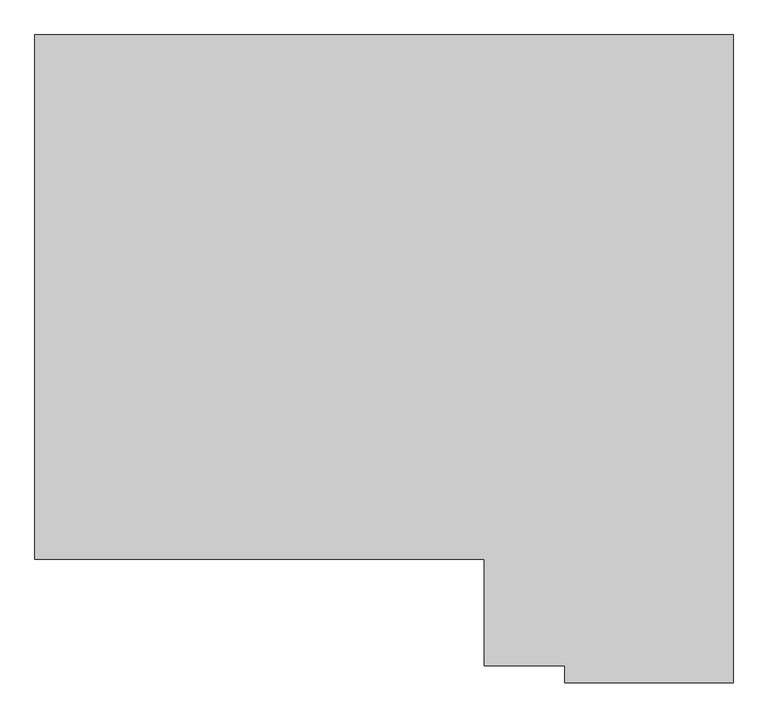
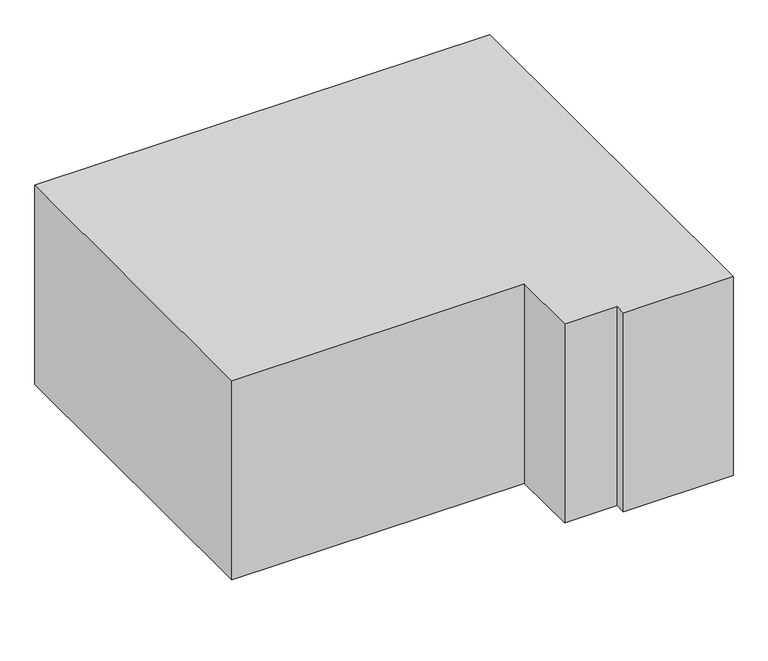
"""IFC4 building model written with IfcOpenShell, lengths in millimetres: proxy geometry, 0_3d."""

from ifc_helpers import new_model, si_unit, origin, origin_with_axes, place, context, project, spatial, polyline, outline, extrude, source, transform, mapped, element, save


def generic_models_ceeb036a(model_context):
    return source(origin(), model_context, "Body", "SweptSolid", [
        extrude(outline(polyline([(6220.0, 5770.0), (6220.0, 0.0), (4720.0, 0.0), (4720.0, 150.0), (4001.4631733, 150.0), (4001.4631733, 1100.0), (0.0, 1100.0), (0.0, 5770.0), (6220.0, 5770.0)])), origin_with_axes(), (0.0, 0.0, 1.0), 2880.0),
    ])


if __name__ == "__main__":
    model = new_model("IFC4")
    model_context = context("Model", 3, world=origin())
    ifc_project = project(units=[si_unit("LENGTHUNIT", "METRE", prefix="MILLI")], contexts=[model_context])
    site = spatial("IfcSite", under=ifc_project)
    building = spatial("IfcBuilding", under=site)
    placement = place(None, origin())
    generic_models_shape = generic_models_ceeb036a(model_context)
    element("IfcBuildingElementProxy", 1, Name="0_3d", ObjectType="0_3d", at=placement, inside=building, context=model_context, shape_type="MappedRepresentation", body=[
        mapped(generic_models_shape, transform((0.0, 0.0, 0.0), x_axis=(1.0, 0.0, 0.0), y_axis=(0.0, 1.0, 0.0), z_axis=(0.0, 0.0, 1.0))),
    ])
    save(model, "model.ifc")

# Revit data of these elements
# Element 1 (IfcBuildingElementProxy, "0_3d")
#   Materials on its faces: "*1"
# Materials
#   "*1": class "Unassigned", colour RGB 175 175 175, transparency 0
